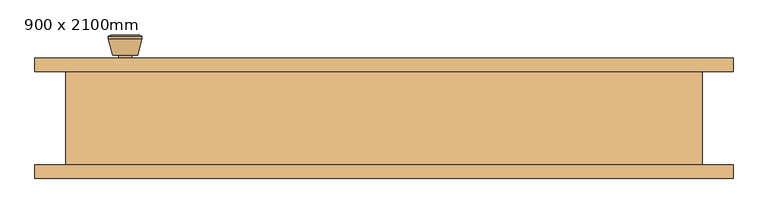
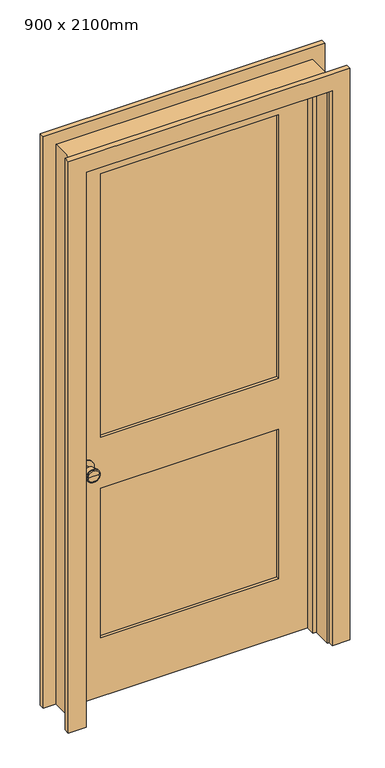
"""IFC4 building model written with IfcOpenShell, lengths in millimetres: door geometry, Porta-Interna-Única-2_Painel-Madeira : 900 x 2100mm."""

from ifc_helpers import new_model, si_unit, point, frame, frame_2d, origin, place, context, project, spatial, polyline, circle_curve, trimmed, segment, composite_curve, outline, extrude, faceted_brep, source, transform, mapped, element, save
from ifc_brep_helpers import plane_surface, cylinder_surface, revolved_surface, advanced_brep


def door_900_x_2100mm_1e3d262a(model_context):
    return source(origin(), model_context, "Body", "SolidModel", [
        advanced_brep(
        [(-386.5, 25.825, 914.4), (-376.5, 25.825, 914.4), (-396.5, 25.825, 914.4), (-366.0241324, -23.175, 914.4), (-386.5, -23.175, 914.4), (-406.9758676, -23.175, 914.4), (-361.5, -21.3471319, 914.4), (-411.5, -21.3471319, 914.4), (-361.5, -17.8834537, 914.4), (-411.5, -17.8834537, 914.4), (-367.863764, 6.825, 914.4), (-405.136236, 6.825, 914.4), (-376.5, 6.825, 914.4), (-396.5, 6.825, 914.4)],
        [
            (0, 1),
            (1, 2, circle_curve(frame((-386.5, 25.825, 914.4), z_axis=(0.0, 1.0, 0.0), x_axis=(-1.0, 0.0, 0.0)), 10.0)),
            (2, 0),
            (2, 1, circle_curve(frame((-386.5, 25.825, 914.4), z_axis=(0.0, 1.0, 0.0), x_axis=(-1.0, 0.0, 0.0)), 10.0)),
            (3, 4),
            (4, 5),
            (5, 3, circle_curve(frame((-386.5, -23.175, 914.4), z_axis=(0.0, -1.0, 0.0), x_axis=(-1.0, 0.0, 0.0)), 20.4758676)),
            (3, 5, circle_curve(frame((-386.5, -23.175, 914.4), z_axis=(0.0, -1.0, 0.0), x_axis=(-1.0, 0.0, 0.0)), 20.4758676)),
            (6, 3),
            (5, 7),
            (7, 6, circle_curve(frame((-386.5, -21.3471319, 914.4), z_axis=(0.0, -1.0, 0.0), x_axis=(-1.0, 0.0, 0.0)), 25.0)),
            (6, 7, circle_curve(frame((-386.5, -21.3471319, 914.4), z_axis=(0.0, -1.0, 0.0), x_axis=(-1.0, 0.0, 0.0)), 25.0)),
            (8, 6),
            (7, 9),
            (9, 8, circle_curve(frame((-386.5, -17.8834537, 914.4), z_axis=(0.0, -1.0, 0.0), x_axis=(-1.0, 0.0, 0.0)), 25.0)),
            (8, 9, circle_curve(frame((-386.5, -17.8834537, 914.4), z_axis=(0.0, -1.0, 0.0), x_axis=(-1.0, 0.0, 0.0)), 25.0)),
            (10, 8),
            (9, 11),
            (11, 10, circle_curve(frame((-386.5, 6.825, 914.4), z_axis=(0.0, -1.0, 0.0), x_axis=(-1.0, 0.0, 0.0)), 18.636236)),
            (10, 11, circle_curve(frame((-386.5, 6.825, 914.4), z_axis=(0.0, -1.0, 0.0), x_axis=(-1.0, 0.0, 0.0)), 18.636236)),
            (12, 10),
            (11, 13),
            (13, 12, circle_curve(frame((-386.5, 6.825, 914.4), z_axis=(0.0, -1.0, 0.0), x_axis=(-1.0, 0.0, 0.0)), 10.0)),
            (12, 13, circle_curve(frame((-386.5, 6.825, 914.4), z_axis=(0.0, -1.0, 0.0), x_axis=(-1.0, 0.0, 0.0)), 10.0)),
            (1, 12),
            (13, 2),
        ],
        [
            plane_surface(frame((-386.5, 25.825, 914.4), z_axis=(0.0, 1.0, 0.0), x_axis=(-1.0, 0.0, 0.0))),
            plane_surface(frame((-386.5, -23.175, 914.4), z_axis=(0.0, -1.0, 0.0), x_axis=(-1.0, 0.0, 0.0))),
            revolved_surface(polyline([(-406.9758676, -23.175, 914.4), (-411.5, -21.3471319, 914.4)]), (-386.5, 25.825, 914.4), (0.0, 1.0, 0.0)),
            cylinder_surface(frame((-386.5, 25.825, 914.4), z_axis=(0.0, 1.0, 0.0), x_axis=(-1.0, 0.0, 0.0)), 25.0),
            revolved_surface(polyline([(-411.5, -17.8834537, 914.4), (-405.136236, 6.825, 914.4)]), (-386.5, 25.825, 914.4), (0.0, 1.0, 0.0)),
            plane_surface(frame((-386.5, 6.825, 914.4), z_axis=(0.0, 1.0, 0.0), x_axis=(-1.0, 0.0, 0.0))),
            cylinder_surface(frame((-386.5, 25.825, 914.4), z_axis=(0.0, 1.0, 0.0), x_axis=(-1.0, 0.0, 0.0)), 10.0),
        ],
        [
            (0, [[1, 2, 3]]),
            (0, [[-3, 4, -1]]),
            (1, [[5, 6, 7]]),
            (1, [[-6, -5, 8]]),
            (2, [[9, -7, 10, 11]]),
            (2, [[-10, -8, -9, 12]]),
            (3, [[13, -11, 14, 15]]),
            (3, [[-14, -12, -13, 16]]),
            (4, [[17, -15, 18, 19]]),
            (4, [[-18, -16, -17, 20]]),
            (5, [[21, -19, 22, 23]]),
            (5, [[-22, -20, -21, 24]]),
            (6, [[25, -23, 26, -2]]),
            (6, [[-26, -24, -25, -4]]),
        ],
    ),
        extrude(outline(composite_curve([segment(trimmed(circle_curve(frame_2d((914.4, -386.5)), 30.0), [point((914.4, -416.5))], [point((914.4, -356.5))], False, "CARTESIAN"), True, "CONTINUOUS"), segment(trimmed(circle_curve(frame_2d((914.4, -386.5)), 30.0), [point((914.4, -356.5))], [point((914.4, -416.5))], False, "CARTESIAN"), True, "CONTINUOUS")], self_intersect=False)), frame((0.0, 25.825, 0.0), z_axis=(0.0, 1.0, 0.0), x_axis=(0.0, 0.0, 1.0)), (0.0, 0.0, 1.0), 6.0),
        advanced_brep(
        [(-386.5, 72.825, 914.4), (-396.5, 72.825, 914.4), (-376.5, 72.825, 914.4), (-366.0241324, 121.825, 914.4), (-406.9758676, 121.825, 914.4), (-386.5, 121.825, 914.4), (-361.5, 119.9971319, 914.4), (-411.5, 119.9971319, 914.4), (-361.5, 116.5334537, 914.4), (-411.5, 116.5334537, 914.4), (-367.863764, 91.825, 914.4), (-405.136236, 91.825, 914.4), (-376.5, 91.825, 914.4), (-396.5, 91.825, 914.4)],
        [
            (0, 1),
            (1, 2, circle_curve(frame((-386.5, 72.825, 914.4), z_axis=(0.0, -1.0, 0.0), x_axis=(-1.0, 0.0, 0.0)), 10.0)),
            (2, 0),
            (2, 1, circle_curve(frame((-386.5, 72.825, 914.4), z_axis=(0.0, -1.0, 0.0), x_axis=(-1.0, 0.0, 0.0)), 10.0)),
            (3, 4, circle_curve(frame((-386.5, 121.825, 914.4), z_axis=(0.0, 1.0, 0.0), x_axis=(-1.0, 0.0, 0.0)), 20.4758676)),
            (4, 5),
            (5, 3),
            (4, 3, circle_curve(frame((-386.5, 121.825, 914.4), z_axis=(0.0, 1.0, 0.0), x_axis=(-1.0, 0.0, 0.0)), 20.4758676)),
            (6, 7, circle_curve(frame((-386.5, 119.9971319, 914.4), z_axis=(0.0, 1.0, 0.0), x_axis=(-1.0, 0.0, 0.0)), 25.0)),
            (7, 4),
            (3, 6),
            (7, 6, circle_curve(frame((-386.5, 119.9971319, 914.4), z_axis=(0.0, 1.0, 0.0), x_axis=(-1.0, 0.0, 0.0)), 25.0)),
            (8, 9, circle_curve(frame((-386.5, 116.5334537, 914.4), z_axis=(0.0, 1.0, 0.0), x_axis=(-1.0, 0.0, 0.0)), 25.0)),
            (9, 7),
            (6, 8),
            (9, 8, circle_curve(frame((-386.5, 116.5334537, 914.4), z_axis=(0.0, 1.0, 0.0), x_axis=(-1.0, 0.0, 0.0)), 25.0)),
            (10, 11, circle_curve(frame((-386.5, 91.825, 914.4), z_axis=(0.0, 1.0, 0.0), x_axis=(-1.0, 0.0, 0.0)), 18.636236)),
            (11, 9),
            (8, 10),
            (11, 10, circle_curve(frame((-386.5, 91.825, 914.4), z_axis=(0.0, 1.0, 0.0), x_axis=(-1.0, 0.0, 0.0)), 18.636236)),
            (12, 13, circle_curve(frame((-386.5, 91.825, 914.4), z_axis=(0.0, 1.0, 0.0), x_axis=(-1.0, 0.0, 0.0)), 10.0)),
            (13, 11),
            (10, 12),
            (13, 12, circle_curve(frame((-386.5, 91.825, 914.4), z_axis=(0.0, 1.0, 0.0), x_axis=(-1.0, 0.0, 0.0)), 10.0)),
            (1, 13),
            (12, 2),
        ],
        [
            plane_surface(frame((-386.5, 72.825, 914.4), z_axis=(0.0, -1.0, 0.0), x_axis=(-1.0, 0.0, 0.0))),
            plane_surface(frame((-386.5, 121.825, 914.4), z_axis=(0.0, 1.0, 0.0), x_axis=(-1.0, 0.0, 0.0))),
            revolved_surface(polyline([(-406.9758676, 121.825, 914.4), (-411.5, 119.9971319, 914.4)]), (-386.5, 72.825, 914.4), (0.0, -1.0, 0.0)),
            cylinder_surface(frame((-386.5, 72.825, 914.4), z_axis=(0.0, -1.0, 0.0), x_axis=(-1.0, 0.0, 0.0)), 25.0),
            revolved_surface(polyline([(-411.5, 116.5334537, 914.4), (-405.136236, 91.825, 914.4)]), (-386.5, 72.825, 914.4), (0.0, -1.0, 0.0)),
            plane_surface(frame((-386.5, 91.825, 914.4), z_axis=(0.0, -1.0, 0.0), x_axis=(-1.0, 0.0, 0.0))),
            cylinder_surface(frame((-386.5, 72.825, 914.4), z_axis=(0.0, -1.0, 0.0), x_axis=(-1.0, 0.0, 0.0)), 10.0),
        ],
        [
            (0, [[1, 2, 3]]),
            (0, [[-3, 4, -1]]),
            (1, [[5, 6, 7]]),
            (1, [[8, -7, -6]]),
            (2, [[9, 10, -5, 11]]),
            (2, [[12, -11, -8, -10]]),
            (3, [[13, 14, -9, 15]]),
            (3, [[16, -15, -12, -14]]),
            (4, [[17, 18, -13, 19]]),
            (4, [[20, -19, -16, -18]]),
            (5, [[21, 22, -17, 23]]),
            (5, [[24, -23, -20, -22]]),
            (6, [[-2, 25, -21, 26]]),
            (6, [[-4, -26, -24, -25]]),
        ],
    ),
        extrude(outline(composite_curve([segment(trimmed(circle_curve(frame_2d((914.4, -386.5)), 30.0), [point((914.4, -416.5))], [point((914.4, -356.5))], False, "CARTESIAN"), True, "CONTINUOUS"), segment(trimmed(circle_curve(frame_2d((914.4, -386.5)), 30.0), [point((914.4, -356.5))], [point((914.4, -416.5))], False, "CARTESIAN"), True, "CONTINUOUS")], self_intersect=False)), frame((0.0, 66.825, 0.0), z_axis=(0.0, 1.0, 0.0), x_axis=(0.0, 0.0, 1.0)), (0.0, 0.0, 1.0), 6.0),
        extrude(outline(polyline([(330.0, 43.4916667), (-330.0, 43.4916667), (-330.0, 55.1583333), (330.0, 55.1583333), (330.0, 43.4916667)])), frame((0.0, 0.0, 1014.4), z_axis=(0.0, 0.0, 1.0), x_axis=(1.0, 0.0, 0.0)), (0.0, 0.0, 1.0), 1030.6),
        extrude(outline(polyline([(330.0, 43.4916667), (-330.0, 43.4916667), (-330.0, 55.1583333), (330.0, 55.1583333), (330.0, 43.4916667)])), frame((0.0, 0.0, 230.0), z_axis=(0.0, 0.0, 1.0), x_axis=(1.0, 0.0, 0.0)), (0.0, 0.0, 1.0), 584.4),
        extrude(outline(polyline([(2165.0, -450.0), (0.0, -450.0), (0.0, 450.0), (2165.0, 450.0), (2165.0, -450.0)]), holes=[polyline([(2045.0, -330.0), (2045.0, 330.0), (1014.4, 330.0), (1014.4, -330.0), (2045.0, -330.0)]), polyline([(814.4, -330.0), (814.4, 330.0), (230.0, 330.0), (230.0, -330.0), (814.4, -330.0)])]), frame((0.0, 31.825, 0.0), z_axis=(0.0, 1.0, 0.0), x_axis=(0.0, 0.0, 1.0)), (0.0, 0.0, 1.0), 35.0),
        faceted_brep([(475.0, 66.825, 0.0), (475.0, -73.175, 0.0), (450.0, -73.175, 0.0), (450.0, -3.1, 0.0), (437.3, -3.1, 0.0), (437.3, 31.825, 0.0), (450.0, 31.825, 0.0), (450.0, 66.825, 0.0), (475.0, 66.825, 2190.0), (475.0, -73.175, 2190.0), (-475.0, -73.175, 2190.0), (-475.0, -73.175, 0.0), (-450.0, -73.175, 0.0), (-450.0, -73.175, 2165.0), (450.0, -73.175, 2165.0), (450.0, -3.1, 2165.0), (-450.0, -3.1, 2165.0), (-450.0, -3.1, 0.0), (-437.3, -3.1, 0.0), (-437.3, -3.1, 2152.3), (437.3, -3.1, 2152.3), (437.3, 31.825, 2152.3), (-437.3, 31.825, 2152.3), (-437.3, 31.825, 0.0), (-450.0, 31.825, 0.0), (-450.0, 31.825, 2165.0), (450.0, 31.825, 2165.0), (450.0, 66.825, 2165.0), (-450.0, 66.825, 2165.0), (-450.0, 66.825, 0.0), (-475.0, 66.825, 0.0), (-475.0, 66.825, 2190.0)], [[[0, 1, 2, 3, 4, 5, 6, 7]], [[1, 0, 8, 9]], [[2, 1, 9, 10, 11, 12, 13, 14]], [[3, 2, 14, 15]], [[4, 3, 15, 16, 17, 18, 19, 20]], [[5, 4, 20, 21]], [[6, 5, 21, 22, 23, 24, 25, 26]], [[7, 6, 26, 27]], [[0, 7, 27, 28, 29, 30, 31, 8]], [[9, 8, 31, 10]], [[15, 14, 13, 16]], [[21, 20, 19, 22]], [[27, 26, 25, 28]], [[30, 29, 24, 23, 18, 17, 12, 11]], [[10, 31, 30, 11]], [[16, 13, 12, 17]], [[22, 19, 18, 23]], [[28, 25, 24, 29]]]),
        extrude(outline(polyline([(0.0, 456.35), (0.0, 521.35), (2236.35, 521.35), (2236.35, -521.35), (0.0, -521.35), (0.0, -456.35), (2171.35, -456.35), (2171.35, 456.35), (0.0, 456.35)])), frame((0.0, -93.175, 0.0), z_axis=(0.0, 1.0, 0.0), x_axis=(0.0, 0.0, 1.0)), (0.0, 0.0, 1.0), 20.0),
        extrude(outline(polyline([(0.0, 456.35), (0.0, 521.35), (2236.35, 521.35), (2236.35, -521.35), (0.0, -521.35), (0.0, -456.35), (2171.35, -456.35), (2171.35, 456.35), (0.0, 456.35)])), frame((0.0, 66.825, 0.0), z_axis=(0.0, 1.0, 0.0), x_axis=(0.0, 0.0, 1.0)), (0.0, 0.0, 1.0), 20.0),
    ])


if __name__ == "__main__":
    model = new_model("IFC4")
    model_context = context("Model", 3, world=origin())
    ifc_project = project(units=[si_unit("LENGTHUNIT", "METRE", prefix="MILLI")], contexts=[model_context])
    site = spatial("IfcSite", under=ifc_project)
    building = spatial("IfcBuilding", under=site)
    placement = place(None, origin())
    door_900_x_2100mm_shape = door_900_x_2100mm_1e3d262a(model_context)
    element("IfcDoor", 1, ObjectType="Porta-Interna-Única-2_Painel-Madeira : 900 x 2100mm", at=placement, inside=building, context=model_context, shape_type="MappedRepresentation", body=[
        mapped(door_900_x_2100mm_shape, transform((0.0, 0.0, 0.0), x_axis=(1.0, 0.0, 0.0), y_axis=(0.0, 1.0, 0.0), z_axis=(0.0, 0.0, 1.0))),
    ])
    save(model, "model.ifc")

# Revit data of these elements
# Type "Porta-Interna-Única-2_Painel-Madeira : 900 x 2100mm"
#   Type Mark = "142"
#   Assembly Code = "C1020300"
#   Analytic Construction = "Madeira"
#   Corrimão superior = 0.120 m
#   Thickness = 0.035 m
#   Thermal Resistance (R) = 0.455703 (m²·K)/W
#   Ângulo de abertura [instance default] = 90.00°
#   Estilos = 0.120 m
#   Rough Width = 0.950 m
#   Rough Height = 2.190 m
#   Bloquear corrimão = 0.200 m
#   Height = 2.165 m
#   Width = 0.900 m
#   Heat Transfer Coefficient (U) = 2.19465 W/(m²·K)
#   Corrimão inferior = 0.230 m
#   Material da apara = Cerejeira
#   Material do painel = Cerejeira
#   Material da moldura = Cerejeira
#   Material da maçaneta = Alumín. 1
#   Visual Light Transmittance = 0
#   Solar Heat Gain Coefficient = 0
#   Wall Closure = (empty or 0)
#   Function = (empty or 0)
# Element 1 (IfcDoor, "Porta-Interna-Única-2_Painel-Madeira : 900 x 2100mm")
#   Materials on its faces: "Cerejeira", "Alumín. 1"
# Materials
#   "Cerejeira": class "Madeira", colour RGB 226 177 128, transparency 0, Description = "Prunus Serotina", Cost = 0
#   "Alumín. 1": class "Metal", colour RGB 247 247 247, transparency 0, Description = "Alumín. 6061", Cost = 0
